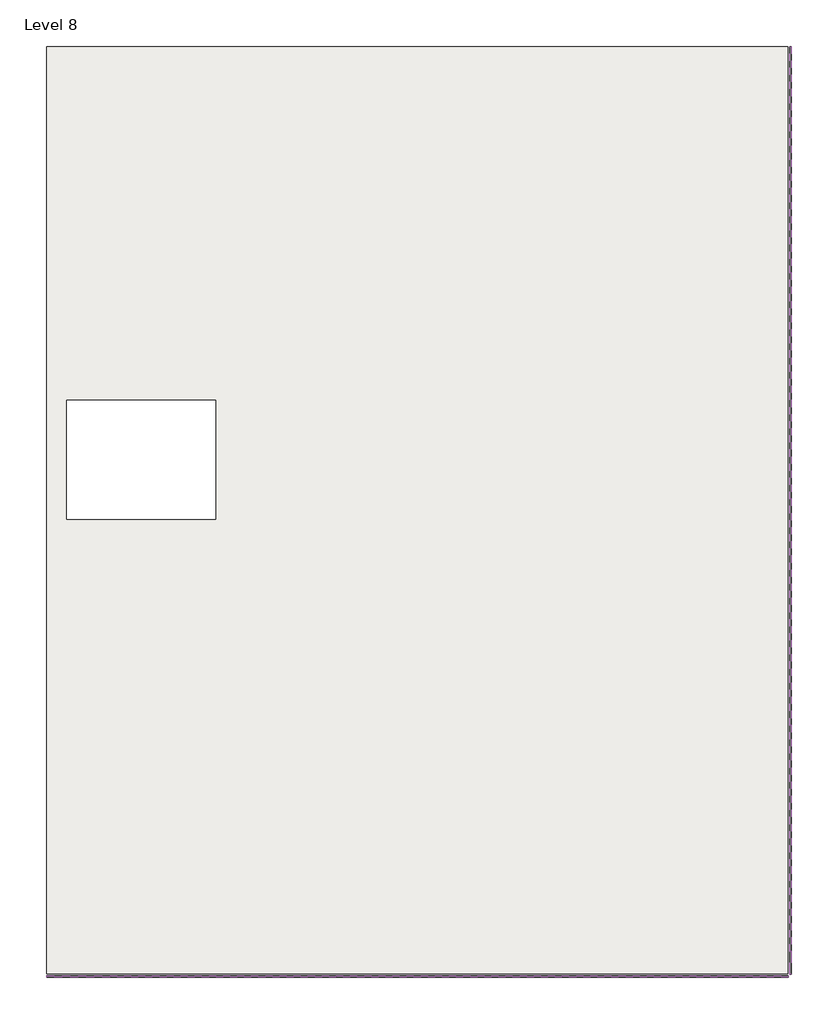
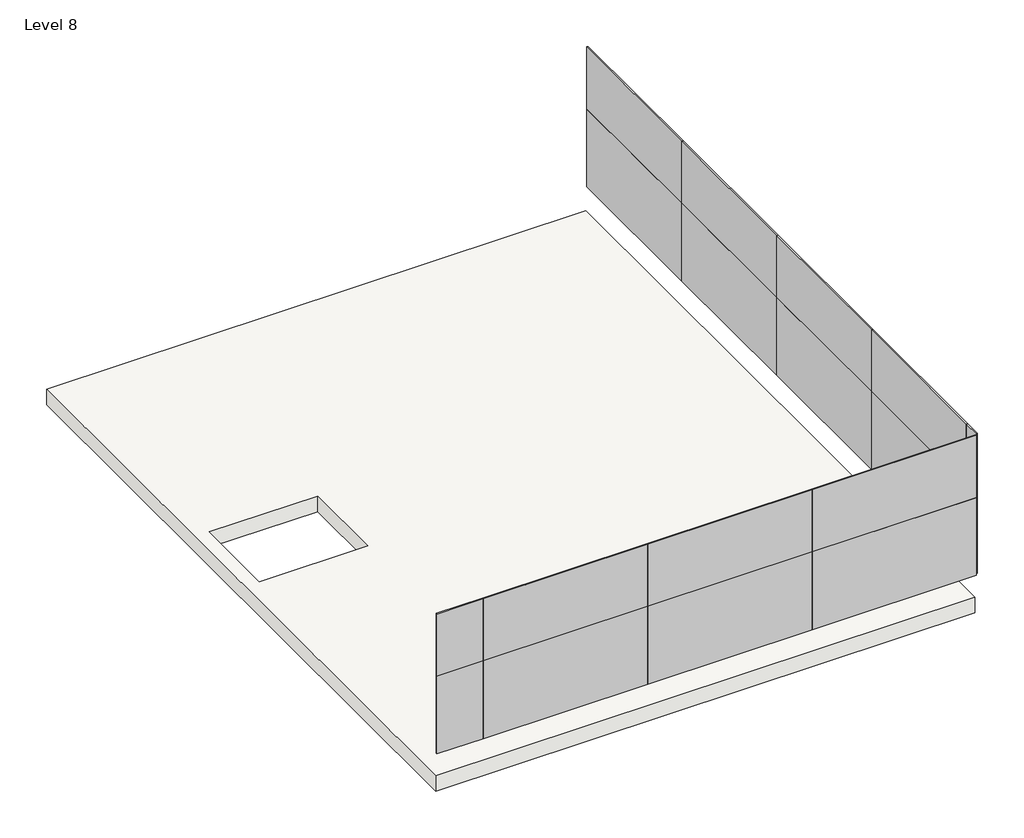
# One storey: 18 plates, 1 slab.
"""IFC4 building model written with IfcOpenShell, lengths in millimetres."""

import ifcopenshell
import ifcopenshell.guid

model = None  # the IFC model being written
_history = None  # IfcOwnerHistory: only IFC2X3 demands one
_inside = {}  # id of a spatial element -> (the spatial element, [elements in it])
_under = {}  # id of a project, library or spatial element -> (it, [spatial elements below it])
_declared = {}  # id of a project -> (the project, [libraries it declares])
_typed = {}  # id of a type object -> (the type object, [elements of that type])
_made_of = {}  # id of a material, layer set ... -> (it, [elements and type objects made of it])


def new_model(schema):
    """Start an empty IFC model of exactly this schema.

    Asked for "IFC4X3", IfcOpenShell would pick the latest addendum, in which some entities
    have other attributes; the version numbers below select the first issue.
    IFC2X3 requires an IfcOwnerHistory on every rooted entity: one is made here for all.
    """
    global model, _history
    if schema == "IFC4X3":
        model = ifcopenshell.file(schema_version=(4, 3, 0, 0))
    else:
        model = ifcopenshell.file(schema=schema)
    _inside.clear()
    _under.clear()
    _declared.clear()
    _typed.clear()
    _made_of.clear()
    _history = None
    if model.schema == "IFC2X3":
        org = make("IfcOrganization", Name="unknown")
        user = make(
            "IfcPersonAndOrganization",
            ThePerson=make("IfcPerson", FamilyName="unknown"),
            TheOrganization=org,
        )
        app = make(
            "IfcApplication",
            ApplicationDeveloper=org,
            Version="unknown",
            ApplicationFullName="unknown",
            ApplicationIdentifier="unknown",
        )
        _history = make(
            "IfcOwnerHistory",
            OwningUser=user,
            OwningApplication=app,
            ChangeAction="ADDED",
            CreationDate=0,
        )
    return model


def make(cls, **values):
    """One entity of the class cls with the attributes given. An attribute that is None is left unset."""
    return model.create_entity(
        cls, **{name: value for name, value in values.items() if value is not None}
    )


def rooted(cls, **values):
    """An entity with a GlobalId (a new one), such as an element, a storey or a relation."""
    return make(cls, GlobalId=ifcopenshell.guid.new(), OwnerHistory=_history, **values)


def si_unit(unit_type, name, prefix=None):
    """IfcSIUnit, for example si_unit("LENGTHUNIT", "METRE", prefix="MILLI")."""
    return make("IfcSIUnit", UnitType=unit_type, Prefix=prefix, Name=name)


def assignment(units):
    """IfcUnitAssignment: the units of a project."""
    return None if units is None else make("IfcUnitAssignment", Units=units)


def point(xyz):
    """IfcCartesianPoint."""
    return None if xyz is None else make("IfcCartesianPoint", Coordinates=xyz)


def direction(xyz):
    """IfcDirection."""
    return None if xyz is None else make("IfcDirection", DirectionRatios=xyz)


def frame(location, z_axis=None, x_axis=None):
    """IfcAxis2Placement3D, a coordinate frame: its origin and axes. An axis left out is left unset."""
    return make(
        "IfcAxis2Placement3D",
        Location=point(location),
        Axis=direction(z_axis),
        RefDirection=direction(x_axis),
    )


def origin():
    """The frame at (0, 0, 0) with its axes left unset."""
    return frame((0.0, 0.0, 0.0))


def origin_with_axes():
    """The frame at (0, 0, 0) with the z axis (0, 0, 1) and the x axis (1, 0, 0) written out."""
    return frame((0.0, 0.0, 0.0), z_axis=(0.0, 0.0, 1.0), x_axis=(1.0, 0.0, 0.0))


def place(relative_to, where):
    """IfcLocalPlacement: puts the frame where relative to a parent placement (None: the world)."""
    return make(
        "IfcLocalPlacement", PlacementRelTo=relative_to, RelativePlacement=where
    )


def context(
    kind, dimensions, precision=None, world=None, true_north=None, identifier=None
):
    """IfcGeometricRepresentationContext, for example the 3D "Model" context."""
    return make(
        "IfcGeometricRepresentationContext",
        ContextIdentifier=identifier,
        ContextType=kind,
        CoordinateSpaceDimension=dimensions,
        Precision=precision,
        WorldCoordinateSystem=world,
        TrueNorth=true_north,
    )


def project(units=None, contexts=None):
    """IfcProject with its units and contexts."""
    return rooted(
        "IfcProject",
        Name="project",
        RepresentationContexts=contexts,
        UnitsInContext=assignment(units),
    )


def spatial(cls, under=None, at=None, **own):
    """A site, building, storey or space (cls), placed at a placement, below another one or the project."""
    s = rooted(cls, ObjectPlacement=at, **own)
    if under is not None:
        _under.setdefault(under.id(), (under, []))[1].append(s)
    return s


def polyline(points):
    """IfcPolyline through the points."""
    return make("IfcPolyline", Points=[point(p) for p in points])


def outline(outer, holes=None, kind="AREA"):
    """IfcArbitraryClosedProfileDef: a profile drawn as a closed curve; with holes, ...WithVoids."""
    if holes is None:
        return make("IfcArbitraryClosedProfileDef", ProfileType=kind, OuterCurve=outer)
    return make(
        "IfcArbitraryProfileDefWithVoids",
        ProfileType=kind,
        OuterCurve=outer,
        InnerCurves=holes,
    )


def extrude(swept, where, along, depth):
    """IfcExtrudedAreaSolid: the profile swept, set in the frame where, extruded along a direction by depth."""
    return make(
        "IfcExtrudedAreaSolid",
        SweptArea=swept,
        Position=where,
        ExtrudedDirection=direction(along),
        Depth=depth,
    )


def shape(context_of_items, identifier, shape_type, items):
    """IfcShapeRepresentation: the items that make up one representation, for example the "Body"."""
    return make(
        "IfcShapeRepresentation",
        ContextOfItems=context_of_items,
        RepresentationIdentifier=identifier,
        RepresentationType=shape_type,
        Items=items,
    )


def source(mapping_origin, context_of_items, identifier, shape_type, items):
    """IfcRepresentationMap: a shape defined once, which mapped items show again and again."""
    return make(
        "IfcRepresentationMap",
        MappingOrigin=mapping_origin,
        MappedRepresentation=shape(context_of_items, identifier, shape_type, items),
    )


def transform(
    local_origin,
    x_axis=None,
    y_axis=None,
    z_axis=None,
    scale=None,
    scale2=None,
    scale3=None,
    uniform=True,
):
    """IfcCartesianTransformationOperator3D, or its non-uniform kind. x_axis, y_axis, z_axis: its Axis1, 2, 3."""
    if uniform:
        return make(
            "IfcCartesianTransformationOperator3D",
            Axis1=direction(x_axis),
            Axis2=direction(y_axis),
            LocalOrigin=point(local_origin),
            Scale=scale,
            Axis3=direction(z_axis),
        )
    return make(
        "IfcCartesianTransformationOperator3DnonUniform",
        Axis1=direction(x_axis),
        Axis2=direction(y_axis),
        LocalOrigin=point(local_origin),
        Scale=scale,
        Axis3=direction(z_axis),
        Scale2=scale2,
        Scale3=scale3,
    )


def mapped(mapping_source, mapping_target):
    """IfcMappedItem: shows the shape of a source again, moved by a transform."""
    return make(
        "IfcMappedItem", MappingSource=mapping_source, MappingTarget=mapping_target
    )


def made_of(thing, what):
    """Note that an element or type object is made of a material, layer set ...; save() writes the relation."""
    if what is not None:
        _made_of.setdefault(what.id(), (what, []))[1].append(thing)
    return thing


def element(
    cls,
    number,
    at=None,
    inside=None,
    cuts=None,
    type_object=None,
    material=None,
    context=None,
    identifier="Body",
    shape_type=None,
    held_by="IfcProductDefinitionShape",
    body=None,
    shapes=None,
    **own,
):
    """One element of the class cls, such as IfcWall. Its Tag is "e" and its number.

    at: its placement. inside: the storey or other place that contains it. cuts: it is an
    opening in that element (IfcRelVoidsElement). A single representation is given by context,
    identifier, shape_type and body (its items); several are given by shapes. held_by: the class
    of the entity that holds the representations. save() writes the other relations.
    """
    e = rooted(cls, Tag="e%d" % number, ObjectPlacement=at, **own)
    if body is not None:
        shapes = [shape(context, identifier, shape_type, body)]
    if shapes is not None:
        e.Representation = make(held_by, Representations=shapes)
    if inside is not None:
        _inside.setdefault(inside.id(), (inside, []))[1].append(e)
    if cuts is not None:
        rooted(
            "IfcRelVoidsElement", RelatingBuildingElement=cuts, RelatedOpeningElement=e
        )
    if type_object is not None:
        _typed.setdefault(type_object.id(), (type_object, []))[1].append(e)
    return made_of(e, material)


def aggregate(whole, parts):
    """IfcRelAggregates: a whole, such as a stair, and the parts it consists of."""
    return rooted("IfcRelAggregates", RelatingObject=whole, RelatedObjects=parts)


def save(model, path):
    """Write the relations noted so far, then the file.

    IfcRelAggregates (storeys below a building ...), IfcRelContainedInSpatialStructure (elements
    in a storey), IfcRelDefinesByType, IfcRelAssociatesMaterial and IfcRelDeclares: one each for
    every whole, place, type object, material and project.
    """
    for whole, parts in _under.values():
        aggregate(whole, parts)
    for where, things in _inside.values():
        rooted(
            "IfcRelContainedInSpatialStructure",
            RelatedElements=things,
            RelatingStructure=where,
        )
    for kind, things in _typed.values():
        rooted("IfcRelDefinesByType", RelatedObjects=things, RelatingType=kind)
    for what, things in _made_of.values():
        rooted("IfcRelAssociatesMaterial", RelatedObjects=things, RelatingMaterial=what)
    for by, libraries in _declared.values():
        rooted("IfcRelDeclares", RelatingContext=by, RelatedDefinitions=libraries)
    model.write(path)


def system_panel_glazed_1e57f9bb(model_context):
    return source(origin(), model_context, "Body", "SweptSolid", [
        extrude(outline(polyline([(1524.0000002, 19.05), (-1524.0000002, 19.05), (-1524.0000002, 44.45), (1524.0000002, 44.45), (1524.0000002, 19.05)])), origin_with_axes(), (0.0, 0.0, 1.0), 1524.0),
    ])


def system_panel_glazed_ccfd9adb(model_context):
    return source(origin(), model_context, "Body", "SweptSolid", [
        extrude(outline(polyline([(427.9999998, 19.05), (-427.9999998, 19.05), (-427.9999998, 44.45), (427.9999998, 44.45), (427.9999998, 19.05)])), origin_with_axes(), (0.0, 0.0, 1.0), 1524.0),
    ])


def system_panel_glazed_efb213d5(model_context):
    return source(origin(), model_context, "Body", "SweptSolid", [
        extrude(outline(polyline([(1524.0000002, 19.05), (-1524.0000002, 19.05), (-1524.0000002, 44.45), (1524.0000002, 44.45), (1524.0000002, 19.05)])), origin_with_axes(), (0.0, 0.0, 1.0), 1216.0),
    ])


def system_panel_glazed_e397b593(model_context):
    return source(origin(), model_context, "Body", "SweptSolid", [
        extrude(outline(polyline([(427.9999998, 19.05), (-427.9999998, 19.05), (-427.9999998, 44.45), (427.9999998, 44.45), (427.9999998, 19.05)])), origin_with_axes(), (0.0, 0.0, 1.0), 1216.0),
    ])


def system_panel_glazed_88f24eba(model_context):
    return source(origin(), model_context, "Body", "SweptSolid", [
        extrude(outline(polyline([(153.9999998, 19.05), (-153.9999998, 19.05), (-153.9999998, 44.45), (153.9999998, 44.45), (153.9999998, 19.05)])), origin_with_axes(), (0.0, 0.0, 1.0), 1524.0),
    ])


def system_panel_glazed_e20ab226(model_context):
    return source(origin(), model_context, "Body", "SweptSolid", [
        extrude(outline(polyline([(153.9999998, 19.05), (-153.9999998, 19.05), (-153.9999998, 44.45), (153.9999998, 44.45), (153.9999998, 19.05)])), origin_with_axes(), (0.0, 0.0, 1.0), 1216.0),
    ])


model = new_model("IFC4")

# Units and contexts
model_context = context("Model", 3, world=origin())
ifc_project = project(units=[si_unit("LENGTHUNIT", "METRE", prefix="MILLI")], contexts=[model_context])

# Site, building, storey
site = spatial("IfcSite", under=ifc_project)
building = spatial("IfcBuilding", under=site)
storey = spatial("IfcBuildingStorey", under=building, Name="Level 8", Elevation=22400.0)

# Plates
placement = place(None, origin())
system_panel_glazed_shape = system_panel_glazed_1e57f9bb(model_context)
element("IfcPlate", 1, ObjectType="System Panel : Glazed", at=placement, inside=storey, context=model_context, shape_type="MappedRepresentation", body=[
    mapped(system_panel_glazed_shape, transform((2137.6340362, 1399.6955828, 22860.0), x_axis=(-1.0, 0.0, 0.0), y_axis=(0.0, -1.0, 0.0), z_axis=(0.0, 0.0, 1.0))),
])
element("IfcPlate", 2, ObjectType="System Panel : Glazed", at=placement, inside=storey, context=model_context, shape_type="MappedRepresentation", body=[
    mapped(system_panel_glazed_shape, transform((-910.3659639, 1399.6955828, 22860.0), x_axis=(-1.0, 0.0, 0.0), y_axis=(0.0, -1.0, 0.0), z_axis=(0.0, 0.0, 1.0))),
])
element("IfcPlate", 3, ObjectType="System Panel : Glazed", at=placement, inside=storey, context=model_context, shape_type="MappedRepresentation", body=[
    mapped(system_panel_glazed_shape, transform((-3958.3659639, 1399.6955828, 22860.0), x_axis=(-1.0, 0.0, 0.0), y_axis=(0.0, -1.0, 0.0), z_axis=(0.0, 0.0, 1.0))),
])
element("IfcPlate", 4, ObjectType="System Panel : Glazed", at=placement, inside=storey, context=model_context, shape_type="MappedRepresentation", body=[
    mapped(system_panel_glazed_shape, transform((3661.6340364, 12375.6955827, 22860.0), x_axis=(0.0, -1.0, 0.0), y_axis=(1.0, 0.0, 0.0), z_axis=(0.0, 0.0, 1.0))),
])
element("IfcPlate", 5, ObjectType="System Panel : Glazed", at=placement, inside=storey, context=model_context, shape_type="MappedRepresentation", body=[
    mapped(system_panel_glazed_shape, transform((3661.6340364, 9327.6955825, 22860.0), x_axis=(0.0, -1.0, 0.0), y_axis=(1.0, 0.0, 0.0), z_axis=(0.0, 0.0, 1.0))),
])
element("IfcPlate", 6, ObjectType="System Panel : Glazed", at=placement, inside=storey, context=model_context, shape_type="MappedRepresentation", body=[
    mapped(system_panel_glazed_shape, transform((3661.6340364, 6279.6955825, 22860.0), x_axis=(0.0, -1.0, 0.0), y_axis=(1.0, 0.0, 0.0), z_axis=(0.0, 0.0, 1.0))),
])
element("IfcPlate", 7, ObjectType="System Panel : Glazed", at=placement, inside=storey, context=model_context, shape_type="MappedRepresentation", body=[
    mapped(system_panel_glazed_shape, transform((3661.6340364, 3231.6955825, 22860.0), x_axis=(0.0, -1.0, 0.0), y_axis=(1.0, 0.0, 0.0), z_axis=(0.0, 0.0, 1.0))),
])
system_panel_glazed_2_shape = system_panel_glazed_ccfd9adb(model_context)
element("IfcPlate", 8, ObjectType="System Panel : Glazed", at=placement, inside=storey, context=model_context, shape_type="MappedRepresentation", body=[
    mapped(system_panel_glazed_2_shape, transform((-5910.3659638, 1399.6955828, 22860.0), x_axis=(-1.0, 0.0, 0.0), y_axis=(0.0, -1.0, 0.0), z_axis=(0.0, 0.0, 1.0))),
])
system_panel_glazed_3_shape = system_panel_glazed_efb213d5(model_context)
element("IfcPlate", 9, ObjectType="System Panel : Glazed", at=placement, inside=storey, context=model_context, shape_type="MappedRepresentation", body=[
    mapped(system_panel_glazed_3_shape, transform((2137.6340362, 1399.6955828, 24384.0), x_axis=(-1.0, 0.0, 0.0), y_axis=(0.0, -1.0, 0.0), z_axis=(0.0, 0.0, 1.0))),
])
element("IfcPlate", 10, ObjectType="System Panel : Glazed", at=placement, inside=storey, context=model_context, shape_type="MappedRepresentation", body=[
    mapped(system_panel_glazed_3_shape, transform((-910.3659639, 1399.6955828, 24384.0), x_axis=(-1.0, 0.0, 0.0), y_axis=(0.0, -1.0, 0.0), z_axis=(0.0, 0.0, 1.0))),
])
element("IfcPlate", 11, ObjectType="System Panel : Glazed", at=placement, inside=storey, context=model_context, shape_type="MappedRepresentation", body=[
    mapped(system_panel_glazed_3_shape, transform((-3958.3659639, 1399.6955828, 24384.0), x_axis=(-1.0, 0.0, 0.0), y_axis=(0.0, -1.0, 0.0), z_axis=(0.0, 0.0, 1.0))),
])
element("IfcPlate", 12, ObjectType="System Panel : Glazed", at=placement, inside=storey, context=model_context, shape_type="MappedRepresentation", body=[
    mapped(system_panel_glazed_3_shape, transform((3661.6340364, 12375.6955827, 24384.0), x_axis=(0.0, -1.0, 0.0), y_axis=(1.0, 0.0, 0.0), z_axis=(0.0, 0.0, 1.0))),
])
element("IfcPlate", 13, ObjectType="System Panel : Glazed", at=placement, inside=storey, context=model_context, shape_type="MappedRepresentation", body=[
    mapped(system_panel_glazed_3_shape, transform((3661.6340364, 9327.6955825, 24384.0), x_axis=(0.0, -1.0, 0.0), y_axis=(1.0, 0.0, 0.0), z_axis=(0.0, 0.0, 1.0))),
])
element("IfcPlate", 14, ObjectType="System Panel : Glazed", at=placement, inside=storey, context=model_context, shape_type="MappedRepresentation", body=[
    mapped(system_panel_glazed_3_shape, transform((3661.6340364, 6279.6955825, 24384.0), x_axis=(0.0, -1.0, 0.0), y_axis=(1.0, 0.0, 0.0), z_axis=(0.0, 0.0, 1.0))),
])
element("IfcPlate", 15, ObjectType="System Panel : Glazed", at=placement, inside=storey, context=model_context, shape_type="MappedRepresentation", body=[
    mapped(system_panel_glazed_3_shape, transform((3661.6340364, 3231.6955825, 24384.0), x_axis=(0.0, -1.0, 0.0), y_axis=(1.0, 0.0, 0.0), z_axis=(0.0, 0.0, 1.0))),
])
system_panel_glazed_4_shape = system_panel_glazed_e397b593(model_context)
element("IfcPlate", 16, ObjectType="System Panel : Glazed", at=placement, inside=storey, context=model_context, shape_type="MappedRepresentation", body=[
    mapped(system_panel_glazed_4_shape, transform((-5910.3659638, 1399.6955828, 24384.0), x_axis=(-1.0, 0.0, 0.0), y_axis=(0.0, -1.0, 0.0), z_axis=(0.0, 0.0, 1.0))),
])
system_panel_glazed_5_shape = system_panel_glazed_88f24eba(model_context)
element("IfcPlate", 17, ObjectType="System Panel : Glazed", at=placement, inside=storey, context=model_context, shape_type="MappedRepresentation", body=[
    mapped(system_panel_glazed_5_shape, transform((3661.6340364, 1553.6955827, 22860.0), x_axis=(0.0, -1.0, 0.0), y_axis=(1.0, 0.0, 0.0), z_axis=(0.0, 0.0, 1.0))),
])
system_panel_glazed_6_shape = system_panel_glazed_e20ab226(model_context)
element("IfcPlate", 18, ObjectType="System Panel : Glazed", at=placement, inside=storey, context=model_context, shape_type="MappedRepresentation", body=[
    mapped(system_panel_glazed_6_shape, transform((3661.6340364, 1553.6955827, 24384.0), x_axis=(0.0, -1.0, 0.0), y_axis=(1.0, 0.0, 0.0), z_axis=(0.0, 0.0, 1.0))),
])

# Slab
element("IfcSlab", 19, ObjectType="Generic - 12\"", at=placement, inside=storey, context=model_context, shape_type="SweptSolid", body=[
    extrude(outline(polyline([(-6335.3659636, 1402.6955828), (-6335.3659636, 13896.6955828), (3658.6340364, 13896.6955828), (3658.6340364, 1402.6955828), (-6335.3659636, 1402.6955828)]), holes=[polyline([(-4059.8993101, 7527.9023719), (-4059.8993101, 9133.9023719), (-6065.8993101, 9133.9023719), (-6065.8993101, 7527.9023719), (-4059.8993101, 7527.9023719)])]), frame((0.0, 0.0, 22095.2), z_axis=(0.0, 0.0, 1.0), x_axis=(1.0, 0.0, 0.0)), (0.0, 0.0, 1.0), 304.8),
])

save(model, "model.ifc")

# Revit data of these elements
# Type "System Panel : Glazed"
#   Construction Type Id = "GSP4R"
#   Analytic Construction = "1/8 in Pilkington single glazing"
#   Visual Light Transmittance = 0.9
#   Solar Heat Gain Coefficient = 0.86
#   Heat Transfer Coefficient (U) = 6.7069 W/(m²·K)
# Type "Generic - 12\""
#   Assembly Code = "B1010"
#   Function = 0
#   Layers, outside or top first: 0.3048 m no material (function 1)
# Elements 1, 2, 3, 4, 5, 6, 7, 8, 9, 10, 11, 12, 13, 14, 15, 16, 17, 18 (IfcPlate, "System Panel : Glazed")
#   Phase Created = New Construction
#   Materials on its faces: "Glass"
# Element 19 (IfcSlab, "Generic - 12\"")
#   built-in parameter 1001955 = -1.5708 (stored number, unit not read)
#   Height Offset From Level = 0.00 m
#   Phase Created = New Construction
#   Materials on its faces: "Default Floor"
# Materials
#   "Glass": class "Glass", colour RGB 0 128 192, transparency 0.75, Description = "Soda Lime Glass", Cost = 0
#   "Default Floor": class "Miscellaneous", colour RGB 128 128 128, transparency 0, Cost = 0
